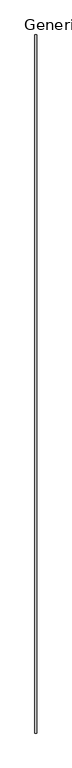
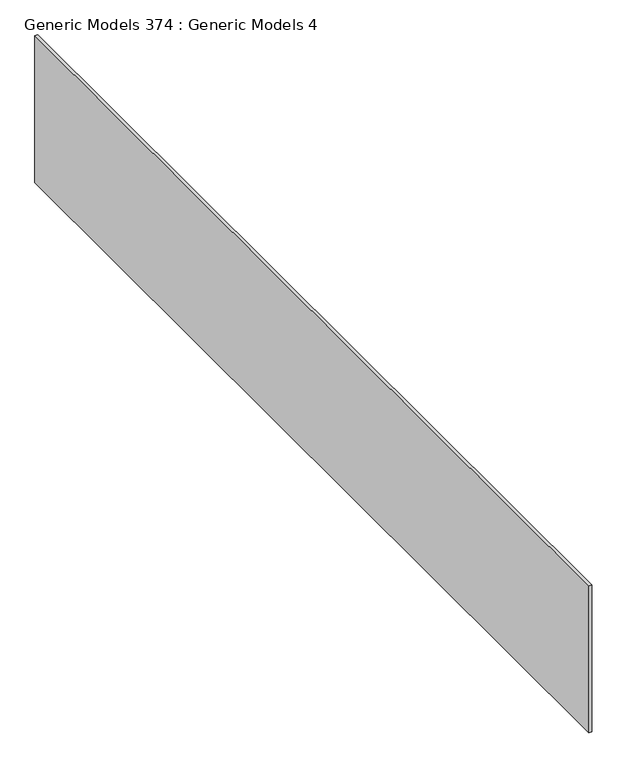
"""IFC4 building model written with IfcOpenShell, lengths in millimetres: proxy geometry, Generic Models 374 : Generic Models 4."""

from ifc_helpers import new_model, si_unit, frame, origin, place, context, project, spatial, polyline, outline, extrude, source, transform, mapped, element, save


def generic_models_374_generic_models_4_0ae622aa(model_context):
    return source(origin(), model_context, "Body", "SweptSolid", [
        extrude(outline(polyline([(-6610.5236296, -6864.9230338), (-6629.5736296, -6864.9230338), (-6629.5736296, -464.1230338), (-6610.5236296, -464.1230338), (-6610.5236296, -6864.9230338)])), frame((0.0, 0.0, 129095.246), z_axis=(0.0, 0.0, 1.0), x_axis=(1.0, 0.0, 0.0)), (0.0, 0.0, 1.0), 1036.7008019),
    ])


if __name__ == "__main__":
    model = new_model("IFC4")
    model_context = context("Model", 3, world=origin())
    ifc_project = project(units=[si_unit("LENGTHUNIT", "METRE", prefix="MILLI")], contexts=[model_context])
    site = spatial("IfcSite", under=ifc_project)
    building = spatial("IfcBuilding", under=site)
    placement = place(None, origin())
    generic_models_374_generic_models_4_shape = generic_models_374_generic_models_4_0ae622aa(model_context)
    element("IfcBuildingElementProxy", 1, Name="Generic Models 374 : Generic Models 4", ObjectType="Generic Models 374 : Generic Models 4", at=placement, inside=building, context=model_context, shape_type="MappedRepresentation", body=[
        mapped(generic_models_374_generic_models_4_shape, transform((0.0, 0.0, 0.0), x_axis=(1.0, 0.0, 0.0), y_axis=(0.0, 1.0, 0.0), z_axis=(0.0, 0.0, 1.0))),
    ])
    save(model, "model.ifc")

# Revit data of these elements
# Element 1 (IfcBuildingElementProxy, "Generic Models 374 : Generic Models 4")
#   Materials on its faces: "_CDX PLYWOOD - SEE STRUCT DWGs"
# Materials
#   "_CDX PLYWOOD - SEE STRUCT DWGs": class "Generic", colour RGB 98 75 74, transparency 0, Cost = 0
